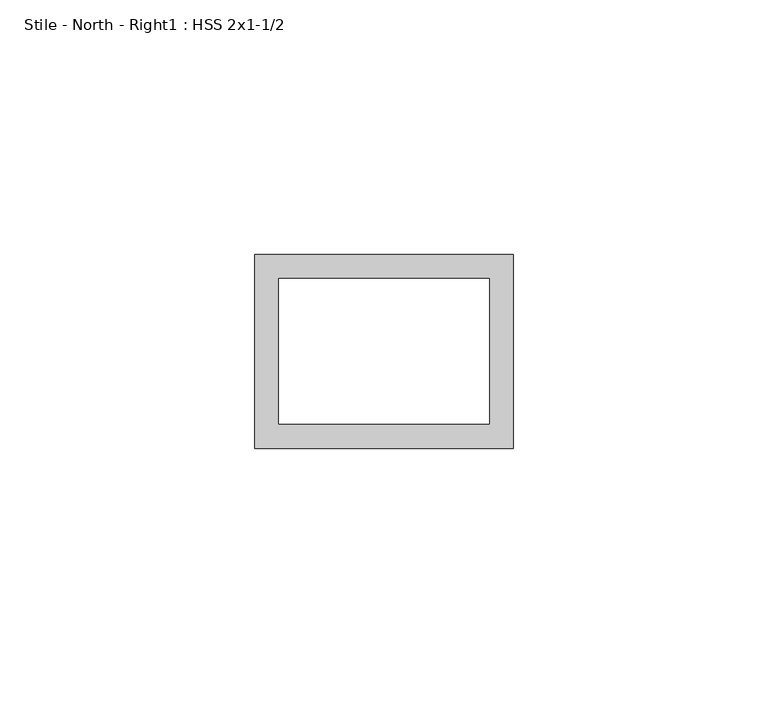
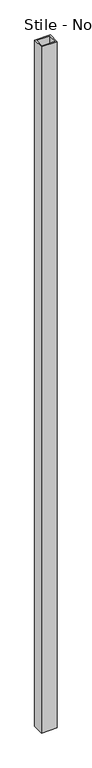
"""IFC4 building model written with IfcOpenShell, lengths in millimetres: proxy geometry, Stile - North - Right1 : HSS 2x1-1/2."""

from ifc_helpers import new_model, si_unit, frame, origin, place, context, project, spatial, polyline, outline, extrude, source, transform, mapped, element, save


def stile_north_right1_hss_2x1_1_2_87095d61(model_context):
    return source(origin(), model_context, "Body", "SweptSolid", [
        extrude(outline(polyline([(587365.8934739, -535163.4663841), (587416.6934739, -535163.4663841), (587416.6934739, -535201.5663841), (587365.8934739, -535201.5663841), (587365.8934739, -535163.4663841)]), holes=[polyline([(587370.6559739, -535168.2288841), (587370.6559739, -535196.8038841), (587411.9309739, -535196.8038841), (587411.9309739, -535168.2288841), (587370.6559739, -535168.2288841)])]), frame((0.0, 0.0, 50.8), z_axis=(0.0, 0.0, 1.0), x_axis=(1.0, 0.0, 0.0)), (0.0, 0.0, 1.0), 2349.5),
    ])


if __name__ == "__main__":
    model = new_model("IFC4")
    model_context = context("Model", 3, world=origin())
    ifc_project = project(units=[si_unit("LENGTHUNIT", "METRE", prefix="MILLI")], contexts=[model_context])
    site = spatial("IfcSite", under=ifc_project)
    building = spatial("IfcBuilding", under=site)
    placement = place(None, origin())
    stile_north_right1_hss_2x1_1_2_shape = stile_north_right1_hss_2x1_1_2_87095d61(model_context)
    element("IfcBuildingElementProxy", 1, Name="Stile - North - Right1 : HSS 2x1-1/2", ObjectType="Stile - North - Right1 : HSS 2x1-1/2", at=placement, inside=building, context=model_context, shape_type="MappedRepresentation", body=[
        mapped(stile_north_right1_hss_2x1_1_2_shape, transform((0.0, 0.0, 0.0), x_axis=(1.0, 0.0, 0.0), y_axis=(0.0, 1.0, 0.0), z_axis=(0.0, 0.0, 1.0))),
    ])
    save(model, "model.ifc")

# Revit data of these elements
# Element 1 (IfcBuildingElementProxy, "Stile - North - Right1 : HSS 2x1-1/2")
#   Materials on its faces: "1-1/2\"X2\" GALV. STL HSS TUBING"
# Materials
#   "1-1/2\"X2\" GALV. STL HSS TUBING": class "Generic", colour RGB 211 211 207, transparency 0, Cost = 0
